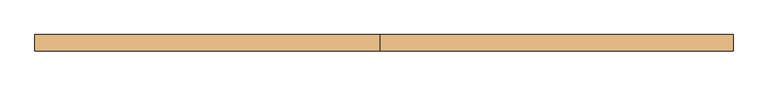
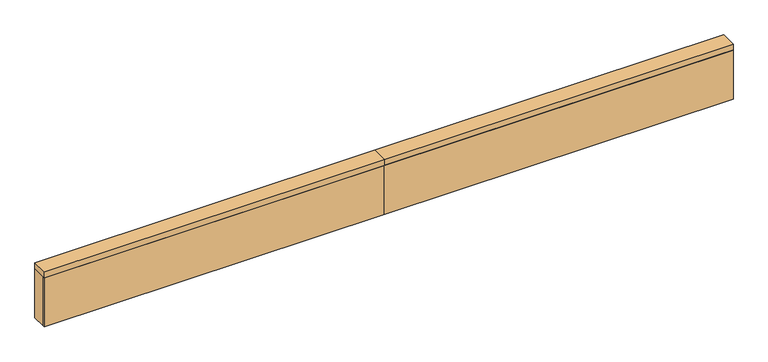
"""IFC4 building model written with IfcOpenShell, lengths in millimetres: door geometry, Schiebetür."""

from ifc_helpers import new_model, si_unit, frame, origin, origin_with_axes, place, context, project, spatial, polyline, outline, extrude, source, transform, mapped, element, save


def door_258b69c4(model_context):
    return source(origin(), model_context, "Body", "SweptSolid", [
        extrude(outline(polyline([(1704.4507425, 6.8571429), (1704.4507425, 0.0), (841.4507425, 0.0), (841.4507425, 6.8571429), (1704.4507425, 6.8571429)])), origin_with_axes(), (0.0, 0.0, 1.0), 128.9099526),
        extrude(outline(polyline([(0.0, 0.0), (0.0, 40.0), (841.4507425, 40.0), (841.4507425, 0.0), (0.0, 0.0)])), frame((0.0, 0.0, 128.9099526), z_axis=(0.0, 0.0, 1.0), x_axis=(1.0, 0.0, 0.0)), (0.0, 0.0, 1.0), 15.4691943),
        extrude(outline(polyline([(12.0, 30.8571429), (12.0, 40.0), (841.4507425, 40.0), (841.4507425, 30.8571429), (12.0, 30.8571429)])), frame((0.0, 0.0, 86.3696682), z_axis=(0.0, 0.0, 1.0), x_axis=(1.0, 0.0, 0.0)), (0.0, 0.0, 1.0), 42.5402844),
        extrude(outline(polyline([(1704.4507425, 40.0), (1704.4507425, 30.8571429), (841.4507425, 30.8571429), (841.4507425, 40.0), (1704.4507425, 40.0)])), frame((0.0, 0.0, 86.3696682), z_axis=(0.0, 0.0, 1.0), x_axis=(1.0, 0.0, 0.0)), (0.0, 0.0, 1.0), 42.5402844),
        extrude(outline(polyline([(1704.4507425, 40.0), (1704.4507425, 0.0), (841.4507425, 0.0), (841.4507425, 40.0), (1704.4507425, 40.0)])), frame((0.0, 0.0, 128.9099526), z_axis=(0.0, 0.0, 1.0), x_axis=(1.0, 0.0, 0.0)), (0.0, 0.0, 1.0), 15.4691943),
        extrude(outline(polyline([(12.0, 6.8571429), (0.0, 6.8571429), (0.0, 40.0), (12.0, 40.0), (12.0, 6.8571429)])), origin_with_axes(), (0.0, 0.0, 1.0), 128.9099526),
        extrude(outline(polyline([(0.0, 0.0), (0.0, 6.8571429), (841.4507425, 6.8571429), (841.4507425, 0.0), (0.0, 0.0)])), origin_with_axes(), (0.0, 0.0, 1.0), 128.9099526),
    ])


if __name__ == "__main__":
    model = new_model("IFC4")
    model_context = context("Model", 3, world=origin())
    ifc_project = project(units=[si_unit("LENGTHUNIT", "METRE", prefix="MILLI")], contexts=[model_context])
    site = spatial("IfcSite", under=ifc_project)
    building = spatial("IfcBuilding", under=site)
    placement = place(None, origin())
    door_shape = door_258b69c4(model_context)
    element("IfcDoor", 1, ObjectType="Schiebetür", at=placement, inside=building, context=model_context, shape_type="MappedRepresentation", body=[
        mapped(door_shape, transform((0.0, 0.0, 0.0), x_axis=(1.0, 0.0, 0.0), y_axis=(0.0, 1.0, 0.0), z_axis=(0.0, 0.0, 1.0))),
    ])
    save(model, "model.ifc")

# Revit data of these elements
# Type "Schiebetür"
#   Type Mark = "50"
# Element 1 (IfcDoor, "Schiebetür")
#   Materials on its faces: "tuer_holzzarge"
# Materials
#   "tuer_holzzarge": class "Unassigned", colour RGB 255 255 255, transparency 0
